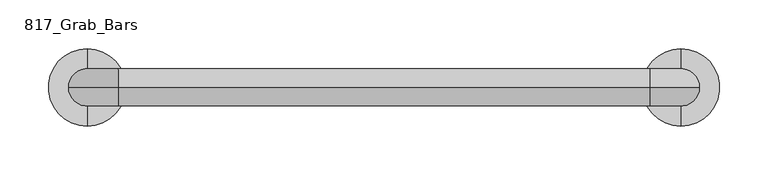
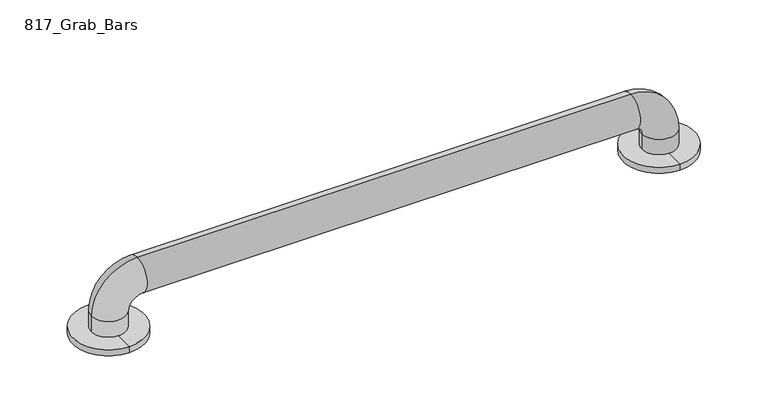
"""IFC4 building model written with IfcOpenShell, lengths in millimetres: proxy geometry, 817_Grab_Bars : 8170-001240."""

from ifc_helpers import new_model, si_unit, point, frame, origin, place, context, project, spatial, circle_curve, ellipse_curve, trimmed, source, transform, mapped, element, save
from ifc_brep_helpers import plane_surface, cylinder_surface, revolved_surface, advanced_brep


def proxy_817_grab_bars_6ffeca21(model_context):
    return source(origin(), model_context, "Body", "AdvancedBrep", [
        advanced_brep(
        [(-211.1375, -496.8875, 7.14375), (-211.1375, -576.2625, 7.14375), (-211.1375, -555.625, 7.14375), (-230.1875, -536.575, 7.14375), (-211.1375, -517.525, 7.14375), (-192.0875, -536.575, 7.14375), (-211.1375, -576.2625, 0.0), (-211.1375, -496.8875, 0.0), (-211.1375, -517.525, 0.0), (-211.1375, -536.575, 0.0), (-211.1375, -555.625, 0.0), (398.4625, -496.8875, 7.14375), (398.4625, -576.2625, 7.14375), (398.4625, -555.625, 7.14375), (379.4125, -536.575, 7.14375), (398.4625, -517.525, 7.14375), (417.5125, -536.575, 7.14375), (398.4625, -576.2625, 0.0), (398.4625, -496.8875, 0.0), (398.4625, -517.525, 0.0), (398.4625, -536.575, 0.0), (398.4625, -555.625, 0.0), (-230.1875, -536.575, 25.4), (-192.0875, -536.575, 25.4), (-179.3875, -536.575, 76.2), (-179.3875, -536.575, 38.1), (366.7125, -536.575, 76.2), (366.7125, -536.575, 38.1), (417.5125, -536.575, 25.4), (379.4125, -536.575, 25.4)],
        [
            (0, 1, circle_curve(frame((-211.1375, -536.575, 7.14375), z_axis=(0.0, 0.0, 1.0), x_axis=(0.0, 1.0, 0.0)), 39.6875)),
            (1, 2),
            (2, 3, circle_curve(frame((-211.1375, -536.575, 7.14375), z_axis=(0.0, 0.0, -1.0), x_axis=(1.0, 0.0, 0.0)), 19.05)),
            (3, 4, circle_curve(frame((-211.1375, -536.575, 7.14375), z_axis=(0.0, 0.0, -1.0), x_axis=(1.0, 0.0, 0.0)), 19.05)),
            (4, 0),
            (1, 0, circle_curve(frame((-211.1375, -536.575, 7.14375), z_axis=(0.0, 0.0, 1.0), x_axis=(0.0, 1.0, 0.0)), 39.6875)),
            (4, 5, circle_curve(frame((-211.1375, -536.575, 7.14375), z_axis=(0.0, 0.0, -1.0), x_axis=(1.0, 0.0, 0.0)), 19.05)),
            (5, 2, circle_curve(frame((-211.1375, -536.575, 7.14375), z_axis=(0.0, 0.0, -1.0), x_axis=(1.0, 0.0, 0.0)), 19.05)),
            (6, 7, circle_curve(frame((-211.1375, -536.575, 0.0), z_axis=(0.0, 0.0, -1.0), x_axis=(0.0, 1.0, 0.0)), 39.6875)),
            (7, 8),
            (8, 9),
            (9, 10),
            (10, 6),
            (7, 6, circle_curve(frame((-211.1375, -536.575, 0.0), z_axis=(0.0, 0.0, -1.0), x_axis=(0.0, 1.0, 0.0)), 39.6875)),
            (0, 7),
            (6, 1),
            (11, 12, circle_curve(frame((398.4625, -536.575, 7.14375), z_axis=(0.0, 0.0, 1.0), x_axis=(0.0, 1.0, 0.0)), 39.6875)),
            (12, 13),
            (13, 14, circle_curve(frame((398.4625, -536.575, 7.14375), z_axis=(0.0, 0.0, -1.0), x_axis=(-1.0, 0.0, 0.0)), 19.05)),
            (14, 15, circle_curve(frame((398.4625, -536.575, 7.14375), z_axis=(0.0, 0.0, -1.0), x_axis=(-1.0, 0.0, 0.0)), 19.05)),
            (15, 11),
            (12, 11, circle_curve(frame((398.4625, -536.575, 7.14375), z_axis=(0.0, 0.0, 1.0), x_axis=(0.0, 1.0, 0.0)), 39.6875)),
            (15, 16, circle_curve(frame((398.4625, -536.575, 7.14375), z_axis=(0.0, 0.0, -1.0), x_axis=(-1.0, 0.0, 0.0)), 19.05)),
            (16, 13, circle_curve(frame((398.4625, -536.575, 7.14375), z_axis=(0.0, 0.0, -1.0), x_axis=(-1.0, 0.0, 0.0)), 19.05)),
            (17, 18, circle_curve(frame((398.4625, -536.575, 0.0), z_axis=(0.0, 0.0, -1.0), x_axis=(0.0, 1.0, 0.0)), 39.6875)),
            (18, 19),
            (19, 20),
            (20, 21),
            (21, 17),
            (18, 17, circle_curve(frame((398.4625, -536.575, 0.0), z_axis=(0.0, 0.0, -1.0), x_axis=(0.0, 1.0, 0.0)), 39.6875)),
            (11, 18),
            (17, 12),
            (22, 23, circle_curve(frame((-211.1375, -536.575, 25.4), z_axis=(0.0, 0.0, -1.0), x_axis=(1.0, 0.0, 0.0)), 19.05)),
            (23, 5),
            (3, 22),
            (23, 22, circle_curve(frame((-211.1375, -536.575, 25.4), z_axis=(0.0, 0.0, -1.0), x_axis=(1.0, 0.0, 0.0)), 19.05)),
            (22, 24, circle_curve(frame((-179.3875, -536.575, 25.4), z_axis=(0.0, 1.0, 0.0), x_axis=(-1.0, 0.0, 0.0)), 50.8)),
            (24, 25, circle_curve(frame((-179.3875, -536.575, 57.15), z_axis=(-1.0, 0.0, 0.0), x_axis=(0.0, 0.0, -1.0)), 19.05)),
            (25, 23, circle_curve(frame((-179.3875, -536.575, 25.4), z_axis=(0.0, -1.0, 0.0), x_axis=(-1.0, 0.0, 0.0)), 12.7)),
            (25, 24, circle_curve(frame((-179.3875, -536.575, 57.15), z_axis=(-1.0, 0.0, 0.0), x_axis=(0.0, 0.0, -1.0)), 19.05)),
            (24, 26),
            (26, 27, circle_curve(frame((366.7125, -536.575, 57.15), z_axis=(-1.0, 0.0, 0.0), x_axis=(0.0, 0.0, -1.0)), 19.05)),
            (27, 25),
            (27, 26, circle_curve(frame((366.7125, -536.575, 57.15), z_axis=(-1.0, 0.0, 0.0), x_axis=(0.0, 0.0, -1.0)), 19.05)),
            (26, 28, circle_curve(frame((366.7125, -536.575, 25.4), z_axis=(0.0, 1.0, 0.0), x_axis=(0.0, 0.0, 1.0)), 50.8)),
            (28, 29, circle_curve(frame((398.4625, -536.575, 25.4), z_axis=(0.0, 0.0, 1.0), x_axis=(-1.0, 0.0, 0.0)), 19.05)),
            (29, 27, circle_curve(frame((366.7125, -536.575, 25.4), z_axis=(0.0, -1.0, 0.0), x_axis=(0.0, 0.0, 1.0)), 12.7)),
            (29, 28, circle_curve(frame((398.4625, -536.575, 25.4), z_axis=(0.0, 0.0, 1.0), x_axis=(-1.0, 0.0, 0.0)), 19.05)),
            (28, 16),
            (14, 29),
        ],
        [
            plane_surface(frame((-211.1375, -536.575, 7.14375), z_axis=(0.0, 0.0, 1.0), x_axis=(0.0, 1.0, 0.0))),
            plane_surface(frame((-211.1375, -536.575, 0.0), z_axis=(0.0, 0.0, -1.0), x_axis=(0.0, 1.0, 0.0))),
            cylinder_surface(frame((-211.1375, -536.575, 7.14375), z_axis=(0.0, 0.0, 1.0), x_axis=(0.0, 1.0, 0.0)), 39.6875),
            plane_surface(frame((398.4625, -536.575, 7.14375), z_axis=(0.0, 0.0, 1.0), x_axis=(0.0, 1.0, 0.0))),
            plane_surface(frame((398.4625, -536.575, 0.0), z_axis=(0.0, 0.0, -1.0), x_axis=(0.0, 1.0, 0.0))),
            cylinder_surface(frame((398.4625, -536.575, 31.75), z_axis=(0.0, 0.0, 1.0), x_axis=(0.0, 1.0, 0.0)), 39.6875),
            cylinder_surface(frame((-211.1375, -536.575, 0.0), z_axis=(0.0, 0.0, -1.0), x_axis=(1.0, 0.0, 0.0)), 19.05),
            revolved_surface(trimmed(ellipse_curve(frame((-211.1375, -536.575, 25.4), z_axis=(0.0, 0.0, -1.0), x_axis=(1.0, 0.0, 0.0)), 19.05, 19.05), [point((-230.1875, -536.575, 25.4))], [point((-192.0875, -536.575, 25.4))], True, "CARTESIAN"), (-179.3875, -536.575, 25.4), (0.0, 1.0, 0.0)),
            revolved_surface(trimmed(ellipse_curve(frame((-211.1375, -536.575, 25.4), z_axis=(0.0, 0.0, -1.0), x_axis=(1.0, 0.0, 0.0)), 19.05, 19.05), [point((-192.0875, -536.575, 25.4))], [point((-230.1875, -536.575, 25.4))], True, "CARTESIAN"), (-179.3875, -536.575, 25.4), (0.0, 1.0, 0.0)),
            cylinder_surface(frame((-179.3875, -536.575, 57.15), z_axis=(-1.0, 0.0, 0.0), x_axis=(0.0, 0.0, -1.0)), 19.05),
            revolved_surface(trimmed(ellipse_curve(frame((366.7125, -536.575, 57.15), z_axis=(-1.0, 0.0, 0.0), x_axis=(0.0, 0.0, -1.0)), 19.05, 19.05), [point((366.7125, -536.575, 76.2))], [point((366.7125, -536.575, 38.1))], True, "CARTESIAN"), (366.7125, -536.575, 25.4), (0.0, 1.0, 0.0)),
            revolved_surface(trimmed(ellipse_curve(frame((366.7125, -536.575, 57.15), z_axis=(-1.0, 0.0, 0.0), x_axis=(0.0, 0.0, -1.0)), 19.05, 19.05), [point((366.7125, -536.575, 38.1))], [point((366.7125, -536.575, 76.2))], True, "CARTESIAN"), (366.7125, -536.575, 25.4), (0.0, 1.0, 0.0)),
            cylinder_surface(frame((398.4625, -536.575, 25.4), z_axis=(0.0, 0.0, 1.0), x_axis=(-1.0, 0.0, 0.0)), 19.05),
        ],
        [
            (0, [[1, 2, 3, 4, 5]]),
            (0, [[6, -5, 7, 8, -2]]),
            (1, [[9, 10, 11, 12, 13]]),
            (1, [[14, -13, -12, -11, -10]]),
            (2, [[-1, 15, -9, 16]]),
            (2, [[-6, -16, -14, -15]]),
            (3, [[17, 18, 19, 20, 21]]),
            (3, [[22, -21, 23, 24, -18]]),
            (4, [[25, 26, 27, 28, 29]]),
            (4, [[30, -29, -28, -27, -26]]),
            (5, [[-17, 31, -25, 32]]),
            (5, [[-22, -32, -30, -31]]),
            (6, [[33, 34, -7, -4, 35]]),
            (6, [[36, -35, -3, -8, -34]]),
            (7, [[-33, 37, 38, 39]]),
            (8, [[-36, -39, 40, -37]]),
            (9, [[-38, 41, 42, 43]]),
            (9, [[-40, -43, 44, -41]]),
            (10, [[-42, 45, 46, 47]]),
            (11, [[-44, -47, 48, -45]]),
            (12, [[-46, 49, -23, -20, 50]]),
            (12, [[-48, -50, -19, -24, -49]]),
        ],
    ),
    ])


if __name__ == "__main__":
    model = new_model("IFC4")
    model_context = context("Model", 3, world=origin())
    ifc_project = project(units=[si_unit("LENGTHUNIT", "METRE", prefix="MILLI")], contexts=[model_context])
    site = spatial("IfcSite", under=ifc_project)
    building = spatial("IfcBuilding", under=site)
    placement = place(None, origin())
    proxy_817_grab_bars_shape = proxy_817_grab_bars_6ffeca21(model_context)
    element("IfcBuildingElementProxy", 1, Name="817_Grab_Bars : 8170-001240", ObjectType="817_Grab_Bars : 8170-001240", at=placement, inside=building, context=model_context, shape_type="MappedRepresentation", body=[
        mapped(proxy_817_grab_bars_shape, transform((0.0, 0.0, 0.0), x_axis=(1.0, 0.0, 0.0), y_axis=(0.0, 1.0, 0.0), z_axis=(0.0, 0.0, 1.0))),
    ])
    save(model, "model.ifc")

# Revit data of these elements
# Type "817_Grab_Bars : 8170-001240"
#   Keynote = "M10281313.01"
#   Warranty Information = "Complete unit, one (1) year"
#   Version = "1.0"
#   Technical Data = "http://www.bradleycorp.com/products/techdata/8815.pdf"
#   URL = "www.bradleycorp.com"
#   Type Comments = "All grab bar configurations are specified using centerline to centerline dimensions."
#   OmniClass Title = ""
#   Modeling Code = ""
#   Model = "8170-001240"
#   Material Note = "FLANGES - 11 GA., TUBING - 18 GA."
#   MasterFormat Section Title = ""
#   Manufacturer = "Bradley Corporation"
#   LEED Credit = ""
#   Instructions [instance default] = "This is a face mounted fixture."
#   Industry Standards = "ANSI Standard A117.1, ADA, ABA, ADAAG, UFAS"
#   Fire Rating = "None"
#   Description = "Grab Bars"
#   Copyright = "This Model Data is Property of Bradley Corporation"
#   Complies to NAFTA = "Yes"
#   Complies To Buy American Act = "Yes"
#   Assembly Code = "C1030200"
#   ADA Compliant = "Yes"
#   Radius = 0' - 0 3/4"
#   Percentage of Recycled Content = 51.67
#   Overall Length = 2' - 3 1/8"
#   OmniClass Number = 0
#   MasterFormat Section Number = 0
#   Length = 2' - 0"
#   Diameter = 0' - 1 1/2"
#   Default Elevation = 2' - 9"
#   Material and Finish = Bradley Corp Stainless Steel - Satin
# Element 1 (IfcBuildingElementProxy, "817_Grab_Bars : 8170-001240")
#   Materials on its faces: "Bradley Corp Stainless Steel - Satin"
# Materials
#   "Bradley Corp Stainless Steel - Satin": class "Metal", colour RGB 189 187 185, transparency 0, Manufacturer = "Bradley Corporation", URL = "www.bradleycorp.com", Description = "Stainless Steel - Satin Finish", Cost = 0
